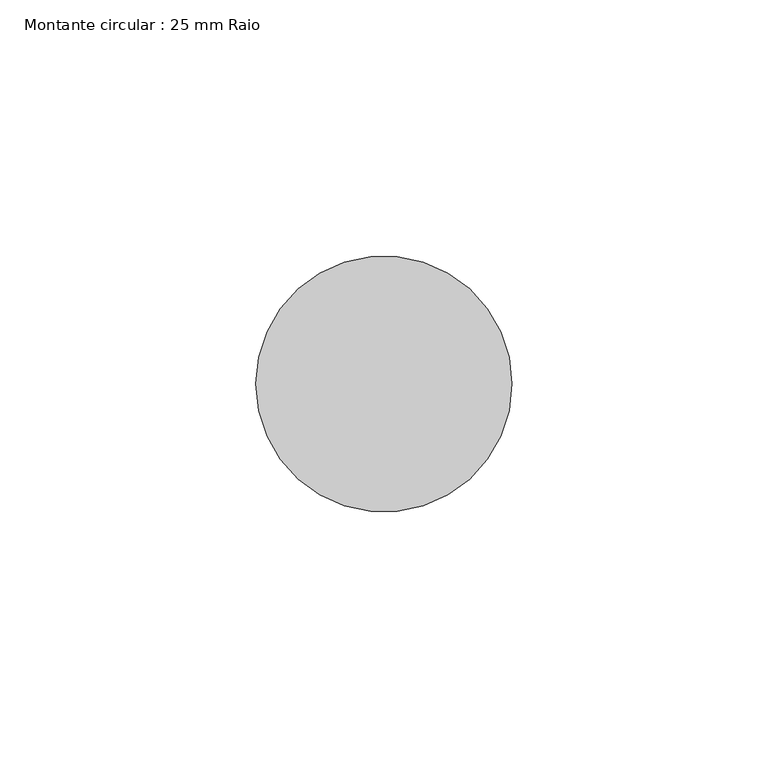
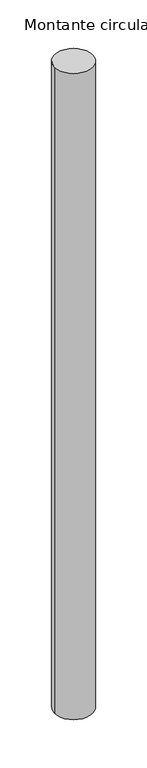
"""IFC4 building model written with IfcOpenShell, lengths in millimetres: member geometry, Montante circular : 25 mm Raio."""

from ifc_helpers import new_model, si_unit, point, frame, frame_2d, origin, place, context, project, spatial, circle_curve, trimmed, segment, composite_curve, outline, extrude, source, transform, mapped, element, save


def montante_circular_25_mm_raio_c63a8114(model_context):
    return source(origin(), model_context, "Body", "SweptSolid", [
        extrude(outline(composite_curve([segment(trimmed(circle_curve(frame_2d((-25.0, 0.0)), 25.0), [point((0.0, 0.0))], [point((-50.0, 0.0))], False, "CARTESIAN"), True, "CONTINUOUS"), segment(trimmed(circle_curve(frame_2d((-25.0, 0.0)), 25.0), [point((-50.0, 0.0))], [point((0.0, 0.0))], False, "CARTESIAN"), True, "CONTINUOUS")], self_intersect=False)), frame((0.0, 0.0, -900.0), z_axis=(0.0, 0.0, 1.0), x_axis=(1.0, 0.0, 0.0)), (0.0, 0.0, 1.0), 900.0),
    ])


if __name__ == "__main__":
    model = new_model("IFC4")
    model_context = context("Model", 3, world=origin())
    ifc_project = project(units=[si_unit("LENGTHUNIT", "METRE", prefix="MILLI")], contexts=[model_context])
    site = spatial("IfcSite", under=ifc_project)
    building = spatial("IfcBuilding", under=site)
    placement = place(None, origin())
    montante_circular_25_mm_raio_shape = montante_circular_25_mm_raio_c63a8114(model_context)
    element("IfcMember", 1, ObjectType="Montante circular : 25 mm Raio", at=placement, inside=building, context=model_context, shape_type="MappedRepresentation", body=[
        mapped(montante_circular_25_mm_raio_shape, transform((0.0, 0.0, 0.0), x_axis=(1.0, 0.0, 0.0), y_axis=(0.0, 1.0, 0.0), z_axis=(0.0, 0.0, 1.0))),
    ])
    save(model, "model.ifc")

# Revit data of these elements
# Type "Montante circular : 25 mm Raio"
#   built-in parameter 1007350 = 0.082021 (stored number, unit not read)
# Element 1 (IfcMember, "Montante circular : 25 mm Raio")
#   Materials on its faces: "Alumín."
# Materials
#   "Alumín.": class "Metal", colour RGB 247 247 247, transparency 0, Description = "Alumín. 6061", Cost = 0
